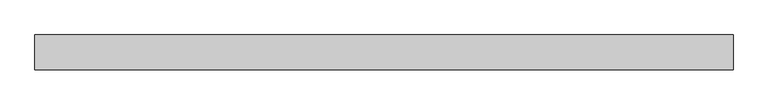
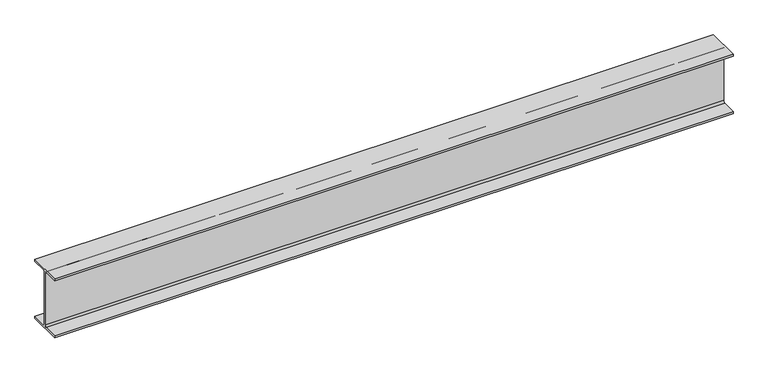
"""IFC4 building model written with IfcOpenShell, lengths in millimetres: beam geometry, Old_Steel Beam_H-KSD3502 : H_SB_ASB_H-200×200x8x12."""

from ifc_helpers import new_model, si_unit, point, frame, frame_2d, origin, place, context, project, spatial, polyline, circle_curve, trimmed, segment, composite_curve, outline, extrude, source, transform, mapped, element, save


def beam_ca562099(model_context):
    return source(origin(), model_context, "Body", "SweptSolid", [
        extrude(outline(composite_curve([segment(polyline([(82.5, -141.5), (82.5, -151.7), (-82.5, -151.7), (-82.5, -141.5), (-11.9, -141.5)]), True, "CONTINUOUS"), segment(trimmed(circle_curve(frame_2d((-11.9, -132.6)), 8.9), [point((-11.9, -141.5))], [point((-3.0, -132.6))], True, "CARTESIAN"), True, "CONTINUOUS"), segment(polyline([(-3.0, -132.6), (-3.0, 132.6)]), True, "CONTINUOUS"), segment(trimmed(circle_curve(frame_2d((-11.9, 132.6)), 8.9), [point((-3.0, 132.6))], [point((-11.9, 141.5))], True, "CARTESIAN"), True, "CONTINUOUS"), segment(polyline([(-11.9, 141.5), (-82.5, 141.5), (-82.5, 151.7), (82.5, 151.7), (82.5, 141.5), (11.9, 141.5)]), True, "CONTINUOUS"), segment(trimmed(circle_curve(frame_2d((11.9, 132.6)), 8.9), [point((11.9, 141.5))], [point((3.0, 132.6))], True, "CARTESIAN"), True, "CONTINUOUS"), segment(polyline([(3.0, 132.6), (3.0, -132.6)]), True, "CONTINUOUS"), segment(trimmed(circle_curve(frame_2d((11.9, -132.6)), 8.9), [point((3.0, -132.6))], [point((11.9, -141.5))], True, "CARTESIAN"), True, "CONTINUOUS"), segment(polyline([(11.9, -141.5), (82.5, -141.5)]), True, "CONTINUOUS")], self_intersect=False)), frame((-1452.9542052, 0.0, 0.0), z_axis=(1.0, 0.0, 0.0), x_axis=(0.0, 1.0, 0.0)), (0.0, 0.0, 1.0), 3291.2393621),
    ])


if __name__ == "__main__":
    model = new_model("IFC4")
    model_context = context("Model", 3, world=origin())
    ifc_project = project(units=[si_unit("LENGTHUNIT", "METRE", prefix="MILLI")], contexts=[model_context])
    site = spatial("IfcSite", under=ifc_project)
    building = spatial("IfcBuilding", under=site)
    placement = place(None, origin())
    beam_shape = beam_ca562099(model_context)
    element("IfcBeam", 1, ObjectType="Old_Steel Beam_H-KSD3502 : H_SB_ASB_H-200×200x8x12", at=placement, inside=building, context=model_context, shape_type="MappedRepresentation", body=[
        mapped(beam_shape, transform((0.0, 0.0, 0.0), x_axis=(1.0, 0.0, 0.0), y_axis=(0.0, 1.0, 0.0), z_axis=(0.0, 0.0, 1.0))),
    ])
    save(model, "model.ifc")

# Revit data of these elements
# Type "Old_Steel Beam_H-KSD3502 : H_SB_ASB_H-200×200x8x12"
#   Width = 20.0 cm
#   Web Thickness = 0.8 cm
#   Web Fillet = 1.3 cm
#   Warping Constant = 141376.0 cm⁶
#   Torsional Moment of Inertia = 26.2485 cm⁴
#   Torsional Modulus = 1.0 cm³
#   Section Area = 63.53 cm²
#   Plastic Modulus weak axis = 244.0 cm³
#   Plastic Modulus strong axis = 525.0 cm³
#   Perimeter = 1.16 m²/m
#   Nominal Weight = 49.90 kgf/m
#   Moment of Inertia weak axis = 1600.00 cm⁴
#   Moment of Inertia strong axis = 4720.00 cm⁴
#   Height = 20.0 cm
#   Flange Thickness = 1.2 cm
#   Elastic Modulus weak axis = 160.0 cm³
#   Elastic Modulus strong axis = 472.0 cm³
#   Centroid Vertical = 10.0 cm
#   Centroid Horizontal = 10.0 cm
#   Length [instance default] = 1.5240 m
#   Structural Material [instance default] = Steel, 45-345
#   Assembly Code = ""
# Element 1 (IfcBeam, "Old_Steel Beam_H-KSD3502 : H_SB_ASB_H-200×200x8x12")
#   Structural Material = none
# Materials
#   "Steel, 45-345": class "Metal", colour RGB 189 187 185, transparency 0, Description = "Steel 345 MPa", Cost = 0
